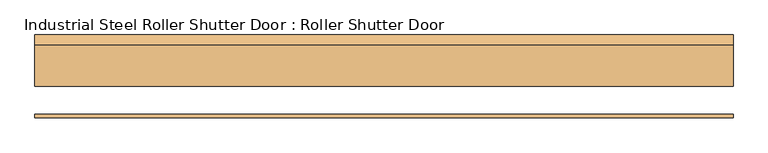
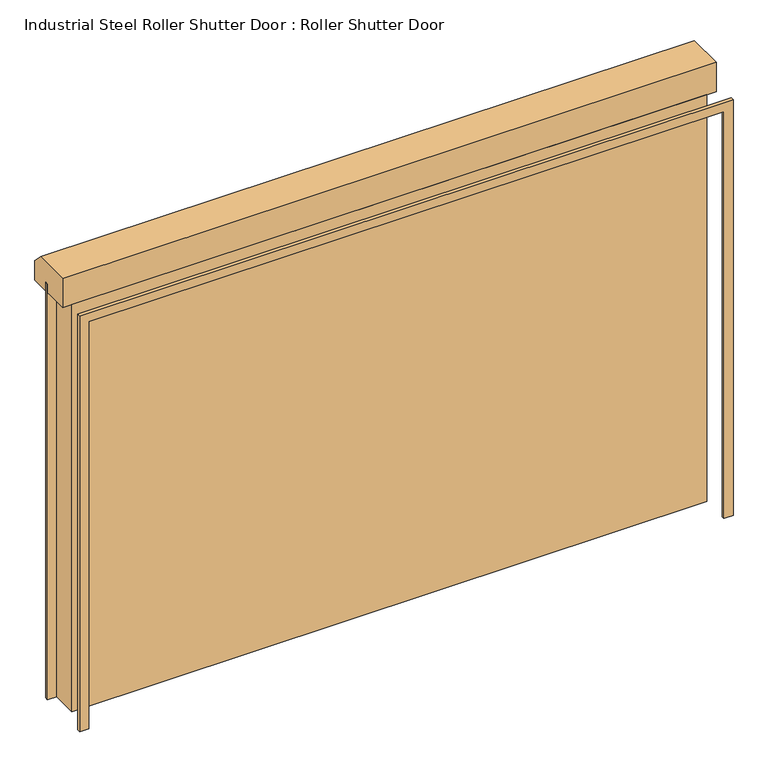
"""IFC4 building model written with IfcOpenShell, lengths in millimetres: door geometry, Industrial Steel Roller Shutter Door : Roller Shutter Door."""

import ifcopenshell
import ifcopenshell.guid

model = None  # the IFC model being written
_history = None  # IfcOwnerHistory: only IFC2X3 demands one
_inside = {}  # id of a spatial element -> (the spatial element, [elements in it])
_under = {}  # id of a project, library or spatial element -> (it, [spatial elements below it])
_declared = {}  # id of a project -> (the project, [libraries it declares])
_typed = {}  # id of a type object -> (the type object, [elements of that type])
_made_of = {}  # id of a material, layer set ... -> (it, [elements and type objects made of it])


def new_model(schema):
    """Start an empty IFC model of exactly this schema.

    Asked for "IFC4X3", IfcOpenShell would pick the latest addendum, in which some entities
    have other attributes; the version numbers below select the first issue.
    IFC2X3 requires an IfcOwnerHistory on every rooted entity: one is made here for all.
    """
    global model, _history
    if schema == "IFC4X3":
        model = ifcopenshell.file(schema_version=(4, 3, 0, 0))
    else:
        model = ifcopenshell.file(schema=schema)
    _inside.clear()
    _under.clear()
    _declared.clear()
    _typed.clear()
    _made_of.clear()
    _history = None
    if model.schema == "IFC2X3":
        org = make("IfcOrganization", Name="unknown")
        user = make(
            "IfcPersonAndOrganization",
            ThePerson=make("IfcPerson", FamilyName="unknown"),
            TheOrganization=org,
        )
        app = make(
            "IfcApplication",
            ApplicationDeveloper=org,
            Version="unknown",
            ApplicationFullName="unknown",
            ApplicationIdentifier="unknown",
        )
        _history = make(
            "IfcOwnerHistory",
            OwningUser=user,
            OwningApplication=app,
            ChangeAction="ADDED",
            CreationDate=0,
        )
    return model


def make(cls, **values):
    """One entity of the class cls with the attributes given. An attribute that is None is left unset."""
    return model.create_entity(
        cls, **{name: value for name, value in values.items() if value is not None}
    )


def rooted(cls, **values):
    """An entity with a GlobalId (a new one), such as an element, a storey or a relation."""
    return make(cls, GlobalId=ifcopenshell.guid.new(), OwnerHistory=_history, **values)


def si_unit(unit_type, name, prefix=None):
    """IfcSIUnit, for example si_unit("LENGTHUNIT", "METRE", prefix="MILLI")."""
    return make("IfcSIUnit", UnitType=unit_type, Prefix=prefix, Name=name)


def assignment(units):
    """IfcUnitAssignment: the units of a project."""
    return None if units is None else make("IfcUnitAssignment", Units=units)


def point(xyz):
    """IfcCartesianPoint."""
    return None if xyz is None else make("IfcCartesianPoint", Coordinates=xyz)


def direction(xyz):
    """IfcDirection."""
    return None if xyz is None else make("IfcDirection", DirectionRatios=xyz)


def frame(location, z_axis=None, x_axis=None):
    """IfcAxis2Placement3D, a coordinate frame: its origin and axes. An axis left out is left unset."""
    return make(
        "IfcAxis2Placement3D",
        Location=point(location),
        Axis=direction(z_axis),
        RefDirection=direction(x_axis),
    )


def origin():
    """The frame at (0, 0, 0) with its axes left unset."""
    return frame((0.0, 0.0, 0.0))


def place(relative_to, where):
    """IfcLocalPlacement: puts the frame where relative to a parent placement (None: the world)."""
    return make(
        "IfcLocalPlacement", PlacementRelTo=relative_to, RelativePlacement=where
    )


def context(
    kind, dimensions, precision=None, world=None, true_north=None, identifier=None
):
    """IfcGeometricRepresentationContext, for example the 3D "Model" context."""
    return make(
        "IfcGeometricRepresentationContext",
        ContextIdentifier=identifier,
        ContextType=kind,
        CoordinateSpaceDimension=dimensions,
        Precision=precision,
        WorldCoordinateSystem=world,
        TrueNorth=true_north,
    )


def project(units=None, contexts=None):
    """IfcProject with its units and contexts."""
    return rooted(
        "IfcProject",
        Name="project",
        RepresentationContexts=contexts,
        UnitsInContext=assignment(units),
    )


def spatial(cls, under=None, at=None, **own):
    """A site, building, storey or space (cls), placed at a placement, below another one or the project."""
    s = rooted(cls, ObjectPlacement=at, **own)
    if under is not None:
        _under.setdefault(under.id(), (under, []))[1].append(s)
    return s


def polyline(points):
    """IfcPolyline through the points."""
    return make("IfcPolyline", Points=[point(p) for p in points])


def outline(outer, holes=None, kind="AREA"):
    """IfcArbitraryClosedProfileDef: a profile drawn as a closed curve; with holes, ...WithVoids."""
    if holes is None:
        return make("IfcArbitraryClosedProfileDef", ProfileType=kind, OuterCurve=outer)
    return make(
        "IfcArbitraryProfileDefWithVoids",
        ProfileType=kind,
        OuterCurve=outer,
        InnerCurves=holes,
    )


def extrude(swept, where, along, depth):
    """IfcExtrudedAreaSolid: the profile swept, set in the frame where, extruded along a direction by depth."""
    return make(
        "IfcExtrudedAreaSolid",
        SweptArea=swept,
        Position=where,
        ExtrudedDirection=direction(along),
        Depth=depth,
    )


def shape(context_of_items, identifier, shape_type, items):
    """IfcShapeRepresentation: the items that make up one representation, for example the "Body"."""
    return make(
        "IfcShapeRepresentation",
        ContextOfItems=context_of_items,
        RepresentationIdentifier=identifier,
        RepresentationType=shape_type,
        Items=items,
    )


def source(mapping_origin, context_of_items, identifier, shape_type, items):
    """IfcRepresentationMap: a shape defined once, which mapped items show again and again."""
    return make(
        "IfcRepresentationMap",
        MappingOrigin=mapping_origin,
        MappedRepresentation=shape(context_of_items, identifier, shape_type, items),
    )


def transform(
    local_origin,
    x_axis=None,
    y_axis=None,
    z_axis=None,
    scale=None,
    scale2=None,
    scale3=None,
    uniform=True,
):
    """IfcCartesianTransformationOperator3D, or its non-uniform kind. x_axis, y_axis, z_axis: its Axis1, 2, 3."""
    if uniform:
        return make(
            "IfcCartesianTransformationOperator3D",
            Axis1=direction(x_axis),
            Axis2=direction(y_axis),
            LocalOrigin=point(local_origin),
            Scale=scale,
            Axis3=direction(z_axis),
        )
    return make(
        "IfcCartesianTransformationOperator3DnonUniform",
        Axis1=direction(x_axis),
        Axis2=direction(y_axis),
        LocalOrigin=point(local_origin),
        Scale=scale,
        Axis3=direction(z_axis),
        Scale2=scale2,
        Scale3=scale3,
    )


def mapped(mapping_source, mapping_target):
    """IfcMappedItem: shows the shape of a source again, moved by a transform."""
    return make(
        "IfcMappedItem", MappingSource=mapping_source, MappingTarget=mapping_target
    )


def made_of(thing, what):
    """Note that an element or type object is made of a material, layer set ...; save() writes the relation."""
    if what is not None:
        _made_of.setdefault(what.id(), (what, []))[1].append(thing)
    return thing


def element(
    cls,
    number,
    at=None,
    inside=None,
    cuts=None,
    type_object=None,
    material=None,
    context=None,
    identifier="Body",
    shape_type=None,
    held_by="IfcProductDefinitionShape",
    body=None,
    shapes=None,
    **own,
):
    """One element of the class cls, such as IfcWall. Its Tag is "e" and its number.

    at: its placement. inside: the storey or other place that contains it. cuts: it is an
    opening in that element (IfcRelVoidsElement). A single representation is given by context,
    identifier, shape_type and body (its items); several are given by shapes. held_by: the class
    of the entity that holds the representations. save() writes the other relations.
    """
    e = rooted(cls, Tag="e%d" % number, ObjectPlacement=at, **own)
    if body is not None:
        shapes = [shape(context, identifier, shape_type, body)]
    if shapes is not None:
        e.Representation = make(held_by, Representations=shapes)
    if inside is not None:
        _inside.setdefault(inside.id(), (inside, []))[1].append(e)
    if cuts is not None:
        rooted(
            "IfcRelVoidsElement", RelatingBuildingElement=cuts, RelatedOpeningElement=e
        )
    if type_object is not None:
        _typed.setdefault(type_object.id(), (type_object, []))[1].append(e)
    return made_of(e, material)


def aggregate(whole, parts):
    """IfcRelAggregates: a whole, such as a stair, and the parts it consists of."""
    return rooted("IfcRelAggregates", RelatingObject=whole, RelatedObjects=parts)


def save(model, path):
    """Write the relations noted so far, then the file.

    IfcRelAggregates (storeys below a building ...), IfcRelContainedInSpatialStructure (elements
    in a storey), IfcRelDefinesByType, IfcRelAssociatesMaterial and IfcRelDeclares: one each for
    every whole, place, type object, material and project.
    """
    for whole, parts in _under.values():
        aggregate(whole, parts)
    for where, things in _inside.values():
        rooted(
            "IfcRelContainedInSpatialStructure",
            RelatedElements=things,
            RelatingStructure=where,
        )
    for kind, things in _typed.values():
        rooted("IfcRelDefinesByType", RelatedObjects=things, RelatingType=kind)
    for what, things in _made_of.values():
        rooted("IfcRelAssociatesMaterial", RelatedObjects=things, RelatingMaterial=what)
    for by, libraries in _declared.values():
        rooted("IfcRelDeclares", RelatingContext=by, RelatedDefinitions=libraries)
    model.write(path)


def industrial_steel_roller_shutter_door_roller_shutter_door_28cb9aac(model_context):
    return source(origin(), model_context, "Body", "SweptSolid", [
        extrude(outline(polyline([(3500.0, -2580.0), (3500.0, 2580.0), (0.0, 2580.0), (0.0, 2655.0), (3575.0, 2655.0), (3575.0, -2655.0), (0.0, -2655.0), (0.0, -2580.0), (3500.0, -2580.0)])), frame((0.0, 215.0, 0.0), z_axis=(0.0, 1.0, 0.0), x_axis=(0.0, 0.0, 1.0)), (0.0, 0.0, 1.0), 25.0),
        extrude(outline(polyline([(3575.0, -2655.0), (0.0, -2655.0), (0.0, -2580.0), (3500.0, -2580.0), (3500.0, 2580.0), (0.0, 2580.0), (0.0, 2655.0), (3575.0, 2655.0), (3575.0, -2655.0)])), frame((0.0, -240.0, 0.0), z_axis=(0.0, 1.0, 0.0), x_axis=(0.0, 0.0, 1.0)), (0.0, 0.0, 1.0), 25.0),
        extrude(outline(polyline([(0.0, 3500.0), (215.0, 3500.0), (215.0, 3475.0), (240.0, 3475.0), (240.0, 0.0), (0.0, 0.0), (0.0, 3500.0)])), frame((-2580.0, 0.0, 0.0), z_axis=(1.0, 0.0, 0.0), x_axis=(0.0, 1.0, 0.0)), (0.0, 0.0, 1.0), 5160.0),
        extrude(outline(polyline([(0.0, 3750.0), (310.0, 3750.0), (390.0, 3670.0), (390.0, 3500.0), (0.0, 3500.0), (0.0, 3750.0)])), frame((-2655.0, 0.0, 0.0), z_axis=(1.0, 0.0, 0.0), x_axis=(0.0, 1.0, 0.0)), (0.0, 0.0, 1.0), 5310.0),
    ])


if __name__ == "__main__":
    model = new_model("IFC4")
    model_context = context("Model", 3, world=origin())
    ifc_project = project(units=[si_unit("LENGTHUNIT", "METRE", prefix="MILLI")], contexts=[model_context])
    site = spatial("IfcSite", under=ifc_project)
    building = spatial("IfcBuilding", under=site)
    placement = place(None, origin())
    industrial_steel_roller_shutter_door_roller_shutter_door_shape = industrial_steel_roller_shutter_door_roller_shutter_door_28cb9aac(model_context)
    element("IfcDoor", 1, ObjectType="Industrial Steel Roller Shutter Door : Roller Shutter Door", at=placement, inside=building, context=model_context, shape_type="MappedRepresentation", body=[
        mapped(industrial_steel_roller_shutter_door_roller_shutter_door_shape, transform((0.0, 0.0, 0.0), x_axis=(1.0, 0.0, 0.0), y_axis=(0.0, 1.0, 0.0), z_axis=(0.0, 0.0, 1.0))),
    ])
    save(model, "model.ifc")

# Revit data of these elements
# Type "Industrial Steel Roller Shutter Door : Roller Shutter Door"
#   Description = "External Roller Shutter Door"
#   Type Mark = "52"
#   Frame Projection Ext. = 25 mm
#   Frame Projection Int. = 25 mm
#   Frame Width = 75 mm
#   Height = 3500 mm
#   Width = 5160 mm
#   Function = (empty or 0)
#   Wall Closure = (empty or 0)
#   Assembly Code = ""
# Element 1 (IfcDoor, "Industrial Steel Roller Shutter Door : Roller Shutter Door")
#   Materials on its faces: "Steel Shutters", "Render 0-255-0"
# Materials
#   "Steel Shutters": class "Vinyl", colour RGB 122 127 125, transparency 0
#   "Render 0-255-0": class "Miscellaneous", colour RGB 0 255 0, transparency 0
